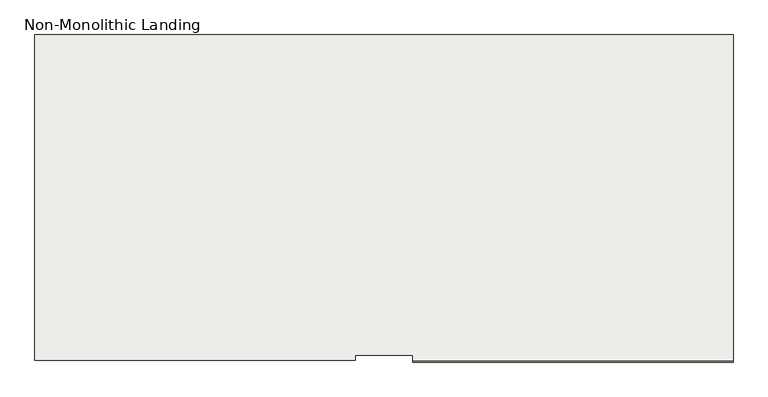
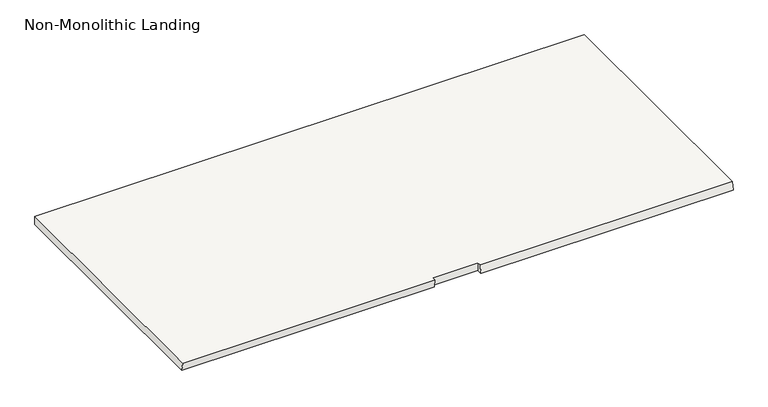
"""IFC4 building model written with IfcOpenShell, lengths in millimetres: slab geometry, Non-Monolithic Landing."""

from ifc_helpers import new_model, si_unit, origin, place, context, project, spatial, faceted_brep, source, transform, mapped, element, save


def non_monolithic_landing_c7120d81(model_context):
    return source(origin(), model_context, "Body", "Brep", [
        faceted_brep([(-226.7120949, 7307.4781803, 17617.6470588), (-226.7120949, 7300.3948469, 17567.6470588), (1293.2879051, 7300.3948469, 17567.6470588), (1293.2879051, 7307.4781803, 17617.6470588), (-499.4393676, 7309.7509075, 17617.6470588), (-499.4393676, 7332.4781803, 17617.6470588), (-226.7120949, 7332.4781803, 17617.6470588), (1293.2879051, 7332.4781803, 17617.6470588), (1293.2879051, 8852.4781803, 17617.6470588), (-2019.4393676, 8852.4781803, 17617.6470588), (-2019.4393676, 7309.7509075, 17617.6470588), (-226.7120949, 7332.4781803, 17567.6470588), (-499.4393676, 7332.4781803, 17567.6470588), (-499.4393676, 7316.8342409, 17567.6470588), (-2019.4393676, 7316.8342409, 17567.6470588), (-2019.4393676, 8852.4781803, 17567.6470588), (1293.2879051, 8852.4781803, 17567.6470588), (1293.2879051, 7332.4781803, 17567.6470588)], [[[0, 1, 2, 3]], [[4, 5, 6, 0, 3, 7, 8, 9, 10]], [[11, 12, 13, 14, 15, 16, 17, 2, 1]], [[5, 4, 13, 12]], [[6, 5, 12, 11]], [[0, 6, 11, 1]], [[7, 3, 2, 17]], [[8, 7, 17, 16]], [[9, 8, 16, 15]], [[10, 9, 15, 14]], [[4, 10, 14, 13]]]),
    ])


if __name__ == "__main__":
    model = new_model("IFC4")
    model_context = context("Model", 3, world=origin())
    ifc_project = project(units=[si_unit("LENGTHUNIT", "METRE", prefix="MILLI")], contexts=[model_context])
    site = spatial("IfcSite", under=ifc_project)
    building = spatial("IfcBuilding", under=site)
    placement = place(None, origin())
    non_monolithic_landing_shape = non_monolithic_landing_c7120d81(model_context)
    element("IfcSlab", 1, ObjectType="Non-Monolithic Landing", at=placement, inside=building, context=model_context, shape_type="MappedRepresentation", body=[
        mapped(non_monolithic_landing_shape, transform((0.0, 0.0, 0.0), x_axis=(1.0, 0.0, 0.0), y_axis=(0.0, 1.0, 0.0), z_axis=(0.0, 0.0, 1.0))),
    ])
    save(model, "model.ifc")
